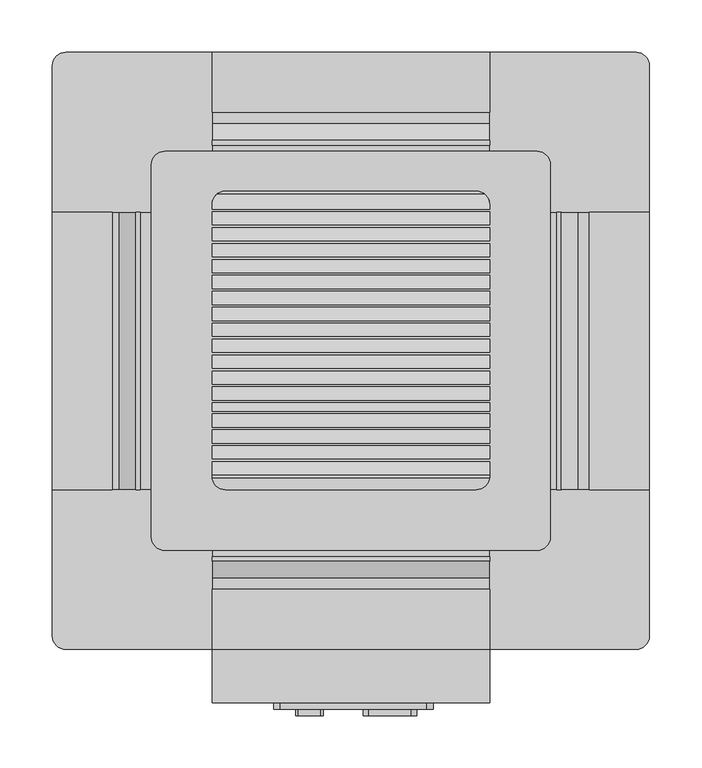
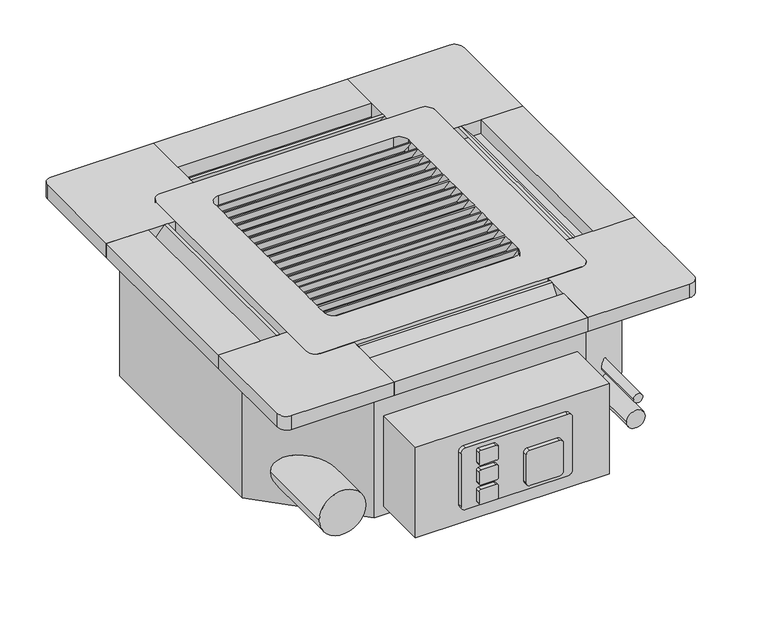
"""IFC4 building model written with IfcOpenShell, lengths in millimetres: proxy geometry, PLFY-P-NCMU-E_4-way_24x24 : PLFY-P12NCMU-E."""

from ifc_helpers import new_model, si_unit, point, frame, frame_2d, origin, place, context, project, spatial, polyline, circle_curve, ellipse_curve, trimmed, segment, composite_curve, outline, extrude, source, transform, mapped, element, save
from ifc_brep_helpers import plane_surface, cylinder_surface, revolved_surface, advanced_brep


def mechanical_equipment_2d84379e(model_context):
    return source(origin(), model_context, "Body", "SolidModel", [
        extrude(outline(polyline([(284.95625, -201.1772913), (227.80625, -201.1772913), (227.80625, 63.9352087), (284.95625, 63.9352087), (284.95625, -201.1772913)])), frame((0.0, 0.0, -1.02e-05), z_axis=(0.0, 0.0, 1.0), x_axis=(1.0, 0.0, 0.0)), (0.0, 0.0, 1.0), 19.84375),
        extrude(outline(polyline([(-284.95625, -201.1772913), (-284.95625, 63.9352087), (-227.80625, 63.9352087), (-227.80625, -201.1772913), (-284.95625, -201.1772913)])), frame((0.0, 0.0, -1.02e-05), z_axis=(0.0, 0.0, 1.0), x_axis=(1.0, 0.0, 0.0)), (0.0, 0.0, 1.0), 19.84375),
        extrude(outline(polyline([(-132.55625, 216.3352087), (132.55625, 216.3352087), (132.55625, 159.1852087), (-132.55625, 159.1852087), (-132.55625, 216.3352087)])), frame((0.0, 0.0, -1.02e-05), z_axis=(0.0, 0.0, 1.0), x_axis=(1.0, 0.0, 0.0)), (0.0, 0.0, 1.0), 19.84375),
        extrude(outline(polyline([(-132.55625, -353.5772913), (-132.55625, -296.4272913), (132.55625, -296.4272913), (132.55625, -353.5772913), (-132.55625, -353.5772913)])), frame((0.0, 0.0, -1.02e-05), z_axis=(0.0, 0.0, 1.0), x_axis=(1.0, 0.0, 0.0)), (0.0, 0.0, 1.0), 19.84375),
        extrude(outline(polyline([(-187.079491, 19.8437398), (-173.1847477, -1.02e-05), (-175.7772913, -1.02e-05), (-189.6720346, 19.8437398), (-187.079491, 19.8437398)])), frame((-132.55625, 0.0, 0.0), z_axis=(1.0, 0.0, 0.0), x_axis=(0.0, 1.0, 0.0)), (0.0, 0.0, 1.0), 265.1125),
        advanced_brep(
        [(-177.8, -259.1210413, -1.02e-05), (-190.5, -246.4210413, -1.02e-05), (-190.5, 109.1789587, -1.02e-05), (-177.8, 121.8789587, -1.02e-05), (177.8, 121.8789587, -1.02e-05), (190.5, 109.1789587, -1.02e-05), (190.5, -246.4210413, -1.02e-05), (177.8, -259.1210413, -1.02e-05), (132.55625, -130.1575084, -1.02e-05), (-132.55625, -130.1575084, -1.02e-05), (-132.55625, -142.7715591, -1.02e-05), (132.55625, -142.7715591, -1.02e-05), (132.55625, -114.9509141, -1.02e-05), (-132.55625, -114.9509141, -1.02e-05), (-132.55625, -127.5649648, -1.02e-05), (132.55625, -127.5649648, -1.02e-05), (132.55625, -104.3814755, -1.02e-05), (-132.55625, -104.3814755, -1.02e-05), (-132.55625, -112.3583705, -1.02e-05), (132.55625, -112.3583705, -1.02e-05), (132.55625, -89.1748812, -1.02e-05), (-132.55625, -89.1748812, -1.02e-05), (-132.55625, -101.7889319, -1.02e-05), (132.55625, -101.7889319, -1.02e-05), (132.55625, -73.9682869, -1.02e-05), (-132.55625, -73.9682869, -1.02e-05), (-132.55625, -86.5823376, -1.02e-05), (132.55625, -86.5823376, -1.02e-05), (132.55625, -58.7616926, -1.02e-05), (-132.55625, -58.7616926, -1.02e-05), (-132.55625, -71.3757433, -1.02e-05), (132.55625, -71.3757433, -1.02e-05), (132.55625, -43.5550983, -1.02e-05), (-132.55625, -43.5550983, -1.02e-05), (-132.55625, -56.169149, -1.02e-05), (132.55625, -56.169149, -1.02e-05), (132.55625, -28.348504, -1.02e-05), (-132.55625, -28.348504, -1.02e-05), (-132.55625, -40.9625547, -1.02e-05), (132.55625, -40.9625547, -1.02e-05), (132.55625, -13.1419097, -1.02e-05), (-132.55625, -13.1419097, -1.02e-05), (-132.55625, -25.7559604, -1.02e-05), (132.55625, -25.7559604, -1.02e-05), (132.55625, 32.4778732, -1.02e-05), (-132.55625, 32.4778732, -1.02e-05), (-132.55625, 19.8638225, -1.02e-05), (132.55625, 19.8638225, -1.02e-05), (132.55625, 47.6844675, -1.02e-05), (-132.55625, 47.6844675, -1.02e-05), (-132.55625, 35.0704168, -1.02e-05), (132.55625, 35.0704168, -1.02e-05), (132.55625, 62.8910618, -1.02e-05), (-132.55625, 62.8910618, -1.02e-05), (-132.55625, 50.2770111, -1.02e-05), (132.55625, 50.2770111, -1.02e-05), (132.55625, 2.0646846, -1.02e-05), (-132.55625, 2.0646846, -1.02e-05), (-132.55625, -10.5493661, -1.02e-05), (132.55625, -10.5493661, -1.02e-05), (-132.55625, 4.6572282, -1.02e-05), (132.55625, 4.6572282, -1.02e-05), (132.55625, 17.2712789, -1.02e-05), (-132.55625, 17.2712789, -1.02e-05), (132.55625, 71.0789587, -1.02e-05), (130.4405727, 78.0976561, -1.02e-05), (-130.4405727, 78.0976561, -1.02e-05), (-132.55625, 71.0789587, -1.02e-05), (-132.55625, 65.4836054, -1.02e-05), (132.55625, 65.4836054, -1.02e-05), (-132.55625, -145.3641027, -1.02e-05), (-132.55625, -157.9781534, -1.02e-05), (132.55625, -157.9781534, -1.02e-05), (132.55625, -145.3641027, -1.02e-05), (-132.55625, -188.4772913, -1.02e-05), (-119.85625, -201.1772913, -1.02e-05), (119.85625, -201.1772913, -1.02e-05), (132.55625, -188.4772913, -1.02e-05), (132.55625, -160.570697, -1.02e-05), (-132.55625, -160.570697, -1.02e-05), (119.85625, 83.7789587, -1.02e-05), (-119.85625, 83.7789587, -1.02e-05), (-128.1576984, 80.6901997, -1.02e-05), (128.1576984, 80.6901997, -1.02e-05), (-177.8, -259.1210413, 19.8437398), (177.8, -259.1210413, 19.8437398), (190.5, -246.4210413, 19.8437398), (190.5, 109.1789587, 19.8437398), (177.8, 121.8789587, 19.8437398), (-177.8, 121.8789587, 19.8437398), (-190.5, 109.1789587, 19.8437398), (-190.5, -246.4210413, 19.8437398), (-132.55625, -144.0522517, 19.8437398), (132.55625, -144.0522517, 19.8437398), (132.55625, -156.6663024, 19.8437398), (-132.55625, -156.6663024, 19.8437398), (-132.55625, -128.8456574, 19.8437398), (132.55625, -128.8456574, 19.8437398), (132.55625, -141.4597081, 19.8437398), (-132.55625, -141.4597081, 19.8437398), (-132.55625, -118.2762188, 19.8437398), (132.55625, -118.2762188, 19.8437398), (132.55625, -126.2531138, 19.8437398), (-132.55625, -126.2531138, 19.8437398), (-132.55625, -103.0696245, 19.8437398), (132.55625, -103.0696245, 19.8437398), (132.55625, -115.6836752, 19.8437398), (-132.55625, -115.6836752, 19.8437398), (-132.55625, -87.8630302, 19.8437398), (132.55625, -87.8630302, 19.8437398), (132.55625, -100.4770809, 19.8437398), (-132.55625, -100.4770809, 19.8437398), (-132.55625, -72.6564359, 19.8437398), (132.55625, -72.6564359, 19.8437398), (132.55625, -85.2704866, 19.8437398), (-132.55625, -85.2704866, 19.8437398), (-132.55625, -57.4498416, 19.8437398), (132.55625, -57.4498416, 19.8437398), (132.55625, -70.0638923, 19.8437398), (-132.55625, -70.0638923, 19.8437398), (-132.55625, -42.2432473, 19.8437398), (132.55625, -42.2432473, 19.8437398), (132.55625, -54.857298, 19.8437398), (-132.55625, -54.857298, 19.8437398), (-132.55625, -27.036653, 19.8437398), (132.55625, -27.036653, 19.8437398), (132.55625, -39.6507037, 19.8437398), (-132.55625, -39.6507037, 19.8437398), (-132.55625, 18.5831298, 19.8437398), (132.55625, 18.5831298, 19.8437398), (132.55625, 5.9690792, 19.8437398), (-132.55625, 5.9690792, 19.8437398), (-132.55625, 33.7897241, 19.8437398), (132.55625, 33.7897241, 19.8437398), (132.55625, 21.1756735, 19.8437398), (-132.55625, 21.1756735, 19.8437398), (-132.55625, 48.9963184, 19.8437398), (132.55625, 48.9963184, 19.8437398), (132.55625, 36.3822678, 19.8437398), (-132.55625, 36.3822678, 19.8437398), (-132.55625, -11.8300587, 19.8437398), (132.55625, -11.8300587, 19.8437398), (132.55625, -24.4441094, 19.8437398), (-132.55625, -24.4441094, 19.8437398), (132.55625, -9.2375151, 19.8437398), (-132.55625, -9.2375151, 19.8437398), (-132.55625, 3.3765356, 19.8437398), (132.55625, 3.3765356, 19.8437398), (-132.55625, 64.2029127, 19.8437398), (132.55625, 64.2029127, 19.8437398), (132.55625, 51.5888621, 19.8437398), (-132.55625, 51.5888621, 19.8437398), (-132.55625, 71.0789587, 19.8437398), (-119.85625, 83.7789587, 19.8437398), (119.85625, 83.7789587, 19.8437398), (132.55625, 71.0789587, 19.8437398), (132.55625, 66.7954564, 19.8437398), (-132.55625, 66.7954564, 19.8437398), (132.55625, -159.258846, 19.8437398), (132.55625, -171.8728967, 19.8437398), (-132.55625, -171.8728967, 19.8437398), (-132.55625, -159.258846, 19.8437398), (132.55625, -188.4772913, 19.8437398), (119.85625, -201.1772913, 19.8437398), (-119.85625, -201.1772913, 19.8437398), (-132.55625, -188.4772913, 19.8437398), (-132.55625, -174.4654403, 19.8437398), (132.55625, -174.4654403, 19.8437398), (132.55625, 71.0789587, 13.7262645), (132.55625, 71.0789587, 10.0237284), (-132.55625, 71.0789587, 10.0237284), (-132.55625, 71.0789587, 13.7262645)],
        [
            (0, 1, circle_curve(frame((-177.8, -246.4210413, -1.02e-05), z_axis=(0.0, 0.0, -1.0), x_axis=(-1.0, 0.0, 0.0)), 12.7)),
            (1, 2),
            (2, 3, circle_curve(frame((-177.8, 109.1789587, -1.02e-05), z_axis=(0.0, 0.0, -1.0), x_axis=(-1.0, 0.0, 0.0)), 12.7)),
            (3, 4),
            (4, 5, circle_curve(frame((177.8, 109.1789587, -1.02e-05), z_axis=(0.0, 0.0, -1.0), x_axis=(-1.0, 0.0, 0.0)), 12.7)),
            (5, 6),
            (6, 7, circle_curve(frame((177.8, -246.4210413, -1.02e-05), z_axis=(0.0, 0.0, -1.0), x_axis=(-1.0, 0.0, 0.0)), 12.7)),
            (7, 0),
            (8, 9),
            (9, 10),
            (10, 11),
            (11, 8),
            (12, 13),
            (13, 14),
            (14, 15),
            (15, 12),
            (16, 17),
            (17, 18),
            (18, 19),
            (19, 16),
            (20, 21),
            (21, 22),
            (22, 23),
            (23, 20),
            (24, 25),
            (25, 26),
            (26, 27),
            (27, 24),
            (28, 29),
            (29, 30),
            (30, 31),
            (31, 28),
            (32, 33),
            (33, 34),
            (34, 35),
            (35, 32),
            (36, 37),
            (37, 38),
            (38, 39),
            (39, 36),
            (40, 41),
            (41, 42),
            (42, 43),
            (43, 40),
            (44, 45),
            (45, 46),
            (46, 47),
            (47, 44),
            (48, 49),
            (49, 50),
            (50, 51),
            (51, 48),
            (52, 53),
            (53, 54),
            (54, 55),
            (55, 52),
            (56, 57),
            (57, 58),
            (58, 59),
            (59, 56),
            (60, 61),
            (61, 62),
            (62, 63),
            (63, 60),
            (64, 65, circle_curve(frame((119.85625, 71.0789587, -1.02e-05), z_axis=(0.0, 0.0, 1.0), x_axis=(-1.0, 0.0, 0.0)), 12.7)),
            (65, 66),
            (66, 67, circle_curve(frame((-119.85625, 71.0789587, -1.02e-05), z_axis=(0.0, 0.0, 1.0), x_axis=(-1.0, 0.0, 0.0)), 12.7)),
            (67, 68),
            (68, 69),
            (69, 64),
            (70, 71),
            (71, 72),
            (72, 73),
            (73, 70),
            (74, 75, circle_curve(frame((-119.85625, -188.4772913, -1.02e-05), z_axis=(0.0, 0.0, 1.0), x_axis=(-1.0, 0.0, 0.0)), 12.7)),
            (75, 76),
            (76, 77, circle_curve(frame((119.85625, -188.4772913, -1.02e-05), z_axis=(0.0, 0.0, 1.0), x_axis=(-1.0, 0.0, 0.0)), 12.7)),
            (77, 78),
            (78, 79),
            (79, 74),
            (80, 81),
            (81, 82, circle_curve(frame((-119.85625, 71.0789587, -1.02e-05), z_axis=(0.0, 0.0, 1.0), x_axis=(-1.0, 0.0, 0.0)), 12.7)),
            (82, 83),
            (83, 80, circle_curve(frame((119.85625, 71.0789587, -1.02e-05), z_axis=(0.0, 0.0, 1.0), x_axis=(-1.0, 0.0, 0.0)), 12.7)),
            (84, 85),
            (85, 86, circle_curve(frame((177.8, -246.4210413, 19.8437398), z_axis=(0.0, 0.0, 1.0), x_axis=(-1.0, 0.0, 0.0)), 12.7)),
            (86, 87),
            (87, 88, circle_curve(frame((177.8, 109.1789587, 19.8437398), z_axis=(0.0, 0.0, 1.0), x_axis=(-1.0, 0.0, 0.0)), 12.7)),
            (88, 89),
            (89, 90, circle_curve(frame((-177.8, 109.1789587, 19.8437398), z_axis=(0.0, 0.0, 1.0), x_axis=(-1.0, 0.0, 0.0)), 12.7)),
            (90, 91),
            (91, 84, circle_curve(frame((-177.8, -246.4210413, 19.8437398), z_axis=(0.0, 0.0, 1.0), x_axis=(-1.0, 0.0, 0.0)), 12.7)),
            (92, 93),
            (93, 94),
            (94, 95),
            (95, 92),
            (96, 97),
            (97, 98),
            (98, 99),
            (99, 96),
            (100, 101),
            (101, 102),
            (102, 103),
            (103, 100),
            (104, 105),
            (105, 106),
            (106, 107),
            (107, 104),
            (108, 109),
            (109, 110),
            (110, 111),
            (111, 108),
            (112, 113),
            (113, 114),
            (114, 115),
            (115, 112),
            (116, 117),
            (117, 118),
            (118, 119),
            (119, 116),
            (120, 121),
            (121, 122),
            (122, 123),
            (123, 120),
            (124, 125),
            (125, 126),
            (126, 127),
            (127, 124),
            (128, 129),
            (129, 130),
            (130, 131),
            (131, 128),
            (132, 133),
            (133, 134),
            (134, 135),
            (135, 132),
            (136, 137),
            (137, 138),
            (138, 139),
            (139, 136),
            (140, 141),
            (141, 142),
            (142, 143),
            (143, 140),
            (144, 145),
            (145, 146),
            (146, 147),
            (147, 144),
            (148, 149),
            (149, 150),
            (150, 151),
            (151, 148),
            (152, 153, circle_curve(frame((-119.85625, 71.0789587, 19.8437398), z_axis=(0.0, 0.0, -1.0), x_axis=(-1.0, 0.0, 0.0)), 12.7)),
            (153, 154),
            (154, 155, circle_curve(frame((119.85625, 71.0789587, 19.8437398), z_axis=(0.0, 0.0, -1.0), x_axis=(-1.0, 0.0, 0.0)), 12.7)),
            (155, 156),
            (156, 157),
            (157, 152),
            (158, 159),
            (159, 160),
            (160, 161),
            (161, 158),
            (162, 163, circle_curve(frame((119.85625, -188.4772913, 19.8437398), z_axis=(0.0, 0.0, -1.0), x_axis=(-1.0, 0.0, 0.0)), 12.7)),
            (163, 164),
            (164, 165, circle_curve(frame((-119.85625, -188.4772913, 19.8437398), z_axis=(0.0, 0.0, -1.0), x_axis=(-1.0, 0.0, 0.0)), 12.7)),
            (165, 166),
            (166, 167),
            (167, 162),
            (155, 168),
            (168, 156),
            (77, 162),
            (167, 78),
            (169, 64),
            (69, 150),
            (149, 169),
            (61, 144),
            (147, 62),
            (141, 56),
            (59, 142),
            (137, 52),
            (55, 138),
            (133, 48),
            (51, 134),
            (129, 44),
            (47, 130),
            (125, 40),
            (43, 126),
            (121, 36),
            (39, 122),
            (117, 32),
            (35, 118),
            (113, 28),
            (31, 114),
            (109, 24),
            (27, 110),
            (105, 20),
            (23, 106),
            (101, 16),
            (19, 102),
            (97, 12),
            (15, 98),
            (93, 8),
            (11, 94),
            (158, 73),
            (72, 159),
            (169, 65, ellipse_curve(frame((119.85625, 71.0789587, 10.0237284), z_axis=(0.0, 0.8191520442889908, 0.5735764363510476), x_axis=(0.0, -0.5735764363510477, 0.8191520442889908)), 22.1417743, 12.7)),
            (154, 80),
            (83, 168, ellipse_curve(frame((119.85625, 71.0789587, 13.7262645), z_axis=(0.0, -0.8191520442889919, -0.573576436351046), x_axis=(0.0, -0.5735764363510462, 0.8191520442889919)), 22.1417743, 12.7)),
            (153, 81),
            (66, 170, ellipse_curve(frame((-119.85625, 71.0789587, 10.0237284), z_axis=(0.0, 0.8191520442889908, 0.5735764363510476), x_axis=(0.0, -0.5735764363510477, 0.8191520442889908)), 22.1417743, 12.7)),
            (170, 67),
            (152, 171),
            (171, 82, ellipse_curve(frame((-119.85625, 71.0789587, 13.7262645), z_axis=(0.0, -0.8191520442889919, -0.573576436351046), x_axis=(0.0, -0.5735764363510462, 0.8191520442889919)), 22.1417743, 12.7)),
            (157, 171),
            (170, 148),
            (151, 68),
            (165, 74),
            (79, 166),
            (145, 60),
            (63, 146),
            (57, 140),
            (143, 58),
            (53, 136),
            (139, 54),
            (49, 132),
            (135, 50),
            (45, 128),
            (131, 46),
            (41, 124),
            (127, 42),
            (37, 120),
            (123, 38),
            (33, 116),
            (119, 34),
            (29, 112),
            (115, 30),
            (25, 108),
            (111, 26),
            (21, 104),
            (107, 22),
            (17, 100),
            (103, 18),
            (13, 96),
            (99, 14),
            (9, 92),
            (95, 10),
            (70, 161),
            (160, 71),
            (164, 75),
            (163, 76),
            (0, 84),
            (91, 1),
            (90, 2),
            (89, 3),
            (88, 4),
            (87, 5),
            (86, 6),
            (85, 7),
        ],
        [
            plane_surface(frame((132.55625, 71.0789587, -1.02e-05), z_axis=(0.0, 0.0, -1.0), x_axis=(0.0, 1.0, 0.0))),
            plane_surface(frame((132.55625, 71.0789587, 19.8437398), z_axis=(0.0, 0.0, 1.0), x_axis=(0.0, -1.0, 0.0))),
            plane_surface(frame((132.55625, -188.4772913, -1.02e-05), z_axis=(-1.0, 0.0, 0.0), x_axis=(0.0, 0.0, 1.0))),
            revolved_surface(polyline([(107.15625, 71.0789587, 28.161208082030438), (107.15625, 71.0789587, -8.113751282030439)]), (119.85625, 71.0789587, 19.8437398), (0.0, 0.0, 1.0)),
            revolved_surface(polyline([(107.15625, 71.0789587, 31.863744182030462), (107.15625, 71.0789587, -4.411215182030464)]), (119.85625, 71.0789587, 19.8437398), (0.0, 0.0, 1.0)),
            plane_surface(frame((119.85625, 83.7789587, -1.02e-05), z_axis=(0.0, -1.0, 0.0), x_axis=(0.0, 0.0, 1.0))),
            revolved_surface(polyline([(-132.55625, 71.0789587, 28.161208082030438), (-132.55625, 71.0789587, -8.113751282030439)]), (-119.85625, 71.0789587, 19.8437398), (0.0, 0.0, 1.0)),
            revolved_surface(polyline([(-132.55625, 71.0789587, 31.863744182030462), (-132.55625, 71.0789587, -4.411215182030464)]), (-119.85625, 71.0789587, 19.8437398), (0.0, 0.0, 1.0)),
            plane_surface(frame((-132.55625, 71.0789587, -1.02e-05), z_axis=(1.0, 0.0, 0.0), x_axis=(0.0, 0.0, 1.0))),
            revolved_surface(polyline([(-132.55625, -188.4772913, 19.8437398), (-132.55625, -188.4772913, -1.0199999998405929e-05)]), (-119.85625, -188.4772913, 19.8437398), (0.0, 0.0, 1.0)),
            plane_surface(frame((-119.85625, -201.1772913, -1.02e-05), z_axis=(0.0, 1.0, 0.0), x_axis=(0.0, 0.0, 1.0))),
            revolved_surface(polyline([(107.15625, -188.4772913, 19.8437398), (107.15625, -188.4772913, -1.0199999998405929e-05)]), (119.85625, -188.4772913, 19.8437398), (0.0, 0.0, 1.0)),
            cylinder_surface(frame((-177.8, -246.4210413, -1.02e-05), z_axis=(0.0, 0.0, -1.0), x_axis=(-1.0, 0.0, 0.0)), 12.7),
            plane_surface(frame((-190.5, -246.4210413, -1.02e-05), z_axis=(-1.0, 0.0, 0.0), x_axis=(0.0, 0.0, 1.0))),
            cylinder_surface(frame((-177.8, 109.1789587, -1.02e-05), z_axis=(0.0, 0.0, -1.0), x_axis=(-1.0, 0.0, 0.0)), 12.7),
            plane_surface(frame((-177.8, 121.8789587, -1.02e-05), z_axis=(0.0, 1.0, 0.0), x_axis=(0.0, 0.0, 1.0))),
            cylinder_surface(frame((177.8, 109.1789587, -1.02e-05), z_axis=(0.0, 0.0, -1.0), x_axis=(-1.0, 0.0, 0.0)), 12.7),
            plane_surface(frame((190.5, 109.1789587, -1.02e-05), z_axis=(1.0, 0.0, 0.0), x_axis=(0.0, 0.0, 1.0))),
            cylinder_surface(frame((177.8, -246.4210413, -1.02e-05), z_axis=(0.0, 0.0, -1.0), x_axis=(-1.0, 0.0, 0.0)), 12.7),
            plane_surface(frame((177.8, -259.1210413, -1.02e-05), z_axis=(0.0, -1.0, 0.0), x_axis=(0.0, 0.0, 1.0))),
            plane_surface(frame((-132.55625, 66.7954564, 19.8437398), z_axis=(0.0, 0.8191520442889919, 0.573576436351046), x_axis=(1.0, 0.0, 0.0))),
            plane_surface(frame((-132.55625, 78.0976561, -1.02e-05), z_axis=(0.0, -0.8191520442889908, -0.5735764363510476), x_axis=(1.0, 0.0, 0.0))),
            plane_surface(frame((-132.55625, -9.2375151, 19.8437398), z_axis=(0.0, 0.8191520442889919, 0.573576436351046), x_axis=(1.0, 0.0, 0.0))),
            plane_surface(frame((-132.55625, 2.0646846, -1.02e-05), z_axis=(0.0, -0.8191520442889908, -0.5735764363510476), x_axis=(1.0, 0.0, 0.0))),
            plane_surface(frame((-132.55625, 51.5888621, 19.8437398), z_axis=(0.0, 0.8191520442889909, 0.5735764363510475), x_axis=(1.0, 0.0, 0.0))),
            plane_surface(frame((-132.55625, 62.8910618, -1.02e-05), z_axis=(0.0, -0.8191520442889917, -0.5735764363510462), x_axis=(1.0, 0.0, 0.0))),
            plane_surface(frame((-132.55625, 36.3822678, 19.8437398), z_axis=(0.0, 0.8191520442889899, 0.5735764363510489), x_axis=(1.0, 0.0, 0.0))),
            plane_surface(frame((-132.55625, 47.6844675, -1.02e-05), z_axis=(0.0, -0.8191520442889901, -0.5735764363510485), x_axis=(1.0, 0.0, 0.0))),
            plane_surface(frame((-132.55625, 21.1756735, 19.8437398), z_axis=(0.0, 0.8191520442889908, 0.5735764363510477), x_axis=(1.0, 0.0, 0.0))),
            plane_surface(frame((-132.55625, 32.4778732, -1.02e-05), z_axis=(0.0, -0.8191520442889919, -0.5735764363510462), x_axis=(1.0, 0.0, 0.0))),
            plane_surface(frame((-132.55625, 5.9690792, 19.8437398), z_axis=(0.0, 0.8191520442889905, 0.5735764363510482), x_axis=(1.0, 0.0, 0.0))),
            plane_surface(frame((-132.55625, 17.2712789, -1.02e-05), z_axis=(0.0, -0.8191520442889922, -0.5735764363510455), x_axis=(1.0, 0.0, 0.0))),
            plane_surface(frame((-132.55625, -24.4441094, 19.8437398), z_axis=(0.0, 0.8191520442889909, 0.5735764363510475), x_axis=(1.0, 0.0, 0.0))),
            plane_surface(frame((-132.55625, -13.1419097, -1.02e-05), z_axis=(0.0, -0.8191520442889917, -0.5735764363510462), x_axis=(1.0, 0.0, 0.0))),
            plane_surface(frame((-132.55625, -39.6507037, 19.8437398), z_axis=(0.0, 0.8191520442889902, 0.5735764363510484), x_axis=(1.0, 0.0, 0.0))),
            plane_surface(frame((-132.55625, -28.348504, -1.02e-05), z_axis=(0.0, -0.8191520442889924, -0.5735764363510453), x_axis=(1.0, 0.0, 0.0))),
            plane_surface(frame((-132.55625, -54.857298, 19.8437398), z_axis=(0.0, 0.8191520442889916, 0.5735764363510465), x_axis=(1.0, 0.0, 0.0))),
            plane_surface(frame((-132.55625, -43.5550983, -1.02e-05), z_axis=(0.0, -0.8191520442889911, -0.5735764363510472), x_axis=(1.0, 0.0, 0.0))),
            plane_surface(frame((-132.55625, -70.0638923, 19.8437398), z_axis=(0.0, 0.8191520442889899, 0.5735764363510489), x_axis=(1.0, 0.0, 0.0))),
            plane_surface(frame((-132.55625, -58.7616926, -1.02e-05), z_axis=(0.0, -0.8191520442889901, -0.5735764363510485), x_axis=(1.0, 0.0, 0.0))),
            plane_surface(frame((-132.55625, -85.2704866, 19.8437398), z_axis=(0.0, 0.8191520442889914, 0.5735764363510468), x_axis=(1.0, 0.0, 0.0))),
            plane_surface(frame((-132.55625, -73.9682869, -1.02e-05), z_axis=(0.0, -0.8191520442889915, -0.5735764363510467), x_axis=(1.0, 0.0, 0.0))),
            plane_surface(frame((-132.55625, -100.4770809, 19.8437398), z_axis=(0.0, 0.8191520442889907, 0.5735764363510477), x_axis=(1.0, 0.0, 0.0))),
            plane_surface(frame((-132.55625, -89.1748812, -1.02e-05), z_axis=(0.0, -0.8191520442889921, -0.5735764363510457), x_axis=(1.0, 0.0, 0.0))),
            plane_surface(frame((-132.55625, -115.6836752, 19.8437398), z_axis=(0.0, 0.819152044288992, 0.5735764363510459), x_axis=(1.0, 0.0, 0.0))),
            plane_surface(frame((-132.55625, -104.3814755, -1.02e-05), z_axis=(0.0, -0.8191520442889908, -0.5735764363510476), x_axis=(1.0, 0.0, 0.0))),
            plane_surface(frame((-132.55625, -126.2531138, 19.8437398), z_axis=(0.0, 0.8191520442889881, 0.5735764363510515), x_axis=(1.0, 0.0, 0.0))),
            plane_surface(frame((-132.55625, -114.9509141, -1.02e-05), z_axis=(0.0, -0.8191520442889907, -0.5735764363510477), x_axis=(1.0, 0.0, 0.0))),
            plane_surface(frame((-132.55625, -141.4597081, 19.8437398), z_axis=(0.0, 0.8191520442889891, 0.5735764363510499), x_axis=(1.0, 0.0, 0.0))),
            plane_surface(frame((-132.55625, -130.1575084, -1.02e-05), z_axis=(0.0, -0.819152044288991, -0.5735764363510474), x_axis=(1.0, 0.0, 0.0))),
            plane_surface(frame((-132.55625, -156.6663024, 19.8437398), z_axis=(0.0, 0.8191520442889885, 0.5735764363510508), x_axis=(1.0, 0.0, 0.0))),
            plane_surface(frame((-132.55625, -145.3641027, -1.02e-05), z_axis=(0.0, -0.819152044288991, -0.5735764363510474), x_axis=(1.0, 0.0, 0.0))),
            plane_surface(frame((-132.55625, -171.8728967, 19.8437398), z_axis=(0.0, 0.8191520442889885, 0.5735764363510508), x_axis=(1.0, 0.0, 0.0))),
            plane_surface(frame((-132.55625, -160.570697, -1.02e-05), z_axis=(0.0, -0.819152044288991, -0.5735764363510474), x_axis=(1.0, 0.0, 0.0))),
        ],
        [
            (0, [[1, 2, 3, 4, 5, 6, 7, 8], [9, 10, 11, 12], [13, 14, 15, 16], [17, 18, 19, 20], [21, 22, 23, 24], [25, 26, 27, 28], [29, 30, 31, 32], [33, 34, 35, 36], [37, 38, 39, 40], [41, 42, 43, 44], [45, 46, 47, 48], [49, 50, 51, 52], [53, 54, 55, 56], [57, 58, 59, 60], [61, 62, 63, 64], [65, 66, 67, 68, 69, 70], [71, 72, 73, 74], [75, 76, 77, 78, 79, 80], [81, 82, 83, 84]]),
            (1, [[85, 86, 87, 88, 89, 90, 91, 92], [93, 94, 95, 96], [97, 98, 99, 100], [101, 102, 103, 104], [105, 106, 107, 108], [109, 110, 111, 112], [113, 114, 115, 116], [117, 118, 119, 120], [121, 122, 123, 124], [125, 126, 127, 128], [129, 130, 131, 132], [133, 134, 135, 136], [137, 138, 139, 140], [141, 142, 143, 144], [145, 146, 147, 148], [149, 150, 151, 152], [153, 154, 155, 156, 157, 158], [159, 160, 161, 162], [163, 164, 165, 166, 167, 168]]),
            (2, [[-156, 169, 170]]),
            (2, [[171, -168, 172, -78]]),
            (2, [[173, -70, 174, -150, 175]]),
            (2, [[176, -148, 177, -62]]),
            (2, [[178, -60, 179, -142]]),
            (2, [[180, -56, 181, -138]]),
            (2, [[182, -52, 183, -134]]),
            (2, [[184, -48, 185, -130]]),
            (2, [[186, -44, 187, -126]]),
            (2, [[188, -40, 189, -122]]),
            (2, [[190, -36, 191, -118]]),
            (2, [[192, -32, 193, -114]]),
            (2, [[194, -28, 195, -110]]),
            (2, [[196, -24, 197, -106]]),
            (2, [[198, -20, 199, -102]]),
            (2, [[200, -16, 201, -98]]),
            (2, [[202, -12, 203, -94]]),
            (2, [[204, -73, 205, -159]]),
            (3, [[-65, -173, 206]]),
            (4, [[-155, 207, -84, 208, -169]]),
            (5, [[-81, -207, -154, 209]]),
            (6, [[-67, 210, 211]]),
            (7, [[-153, 212, 213, -82, -209]]),
            (8, [[-158, 214, -212]]),
            (8, [[-211, 215, -152, 216, -68]]),
            (8, [[217, -80, 218, -166]]),
            (8, [[219, -64, 220, -146]]),
            (8, [[221, -144, 222, -58]]),
            (8, [[223, -140, 224, -54]]),
            (8, [[225, -136, 226, -50]]),
            (8, [[227, -132, 228, -46]]),
            (8, [[229, -128, 230, -42]]),
            (8, [[231, -124, 232, -38]]),
            (8, [[233, -120, 234, -34]]),
            (8, [[235, -116, 236, -30]]),
            (8, [[237, -112, 238, -26]]),
            (8, [[239, -108, 240, -22]]),
            (8, [[241, -104, 242, -18]]),
            (8, [[243, -100, 244, -14]]),
            (8, [[245, -96, 246, -10]]),
            (8, [[247, -161, 248, -71]]),
            (9, [[-75, -217, -165, 249]]),
            (10, [[-76, -249, -164, 250]]),
            (11, [[-77, -250, -163, -171]]),
            (12, [[-1, 251, -92, 252]]),
            (13, [[-2, -252, -91, 253]]),
            (14, [[-3, -253, -90, 254]]),
            (15, [[-4, -254, -89, 255]]),
            (16, [[-5, -255, -88, 256]]),
            (17, [[-6, -256, -87, 257]]),
            (18, [[-7, -257, -86, 258]]),
            (19, [[-8, -258, -85, -251]]),
            (20, [[-157, -170, -208, -83, -213, -214]]),
            (21, [[-149, -215, -210, -66, -206, -175]]),
            (22, [[-145, -176, -61, -219]]),
            (23, [[-57, -178, -141, -221]]),
            (24, [[-151, -174, -69, -216]]),
            (25, [[-53, -180, -137, -223]]),
            (26, [[-139, -181, -55, -224]]),
            (27, [[-49, -182, -133, -225]]),
            (28, [[-135, -183, -51, -226]]),
            (29, [[-45, -184, -129, -227]]),
            (30, [[-131, -185, -47, -228]]),
            (31, [[-63, -177, -147, -220]]),
            (32, [[-143, -179, -59, -222]]),
            (33, [[-41, -186, -125, -229]]),
            (34, [[-127, -187, -43, -230]]),
            (35, [[-37, -188, -121, -231]]),
            (36, [[-123, -189, -39, -232]]),
            (37, [[-33, -190, -117, -233]]),
            (38, [[-119, -191, -35, -234]]),
            (39, [[-29, -192, -113, -235]]),
            (40, [[-115, -193, -31, -236]]),
            (41, [[-25, -194, -109, -237]]),
            (42, [[-111, -195, -27, -238]]),
            (43, [[-21, -196, -105, -239]]),
            (44, [[-107, -197, -23, -240]]),
            (45, [[-17, -198, -101, -241]]),
            (46, [[-103, -199, -19, -242]]),
            (47, [[-13, -200, -97, -243]]),
            (48, [[-99, -201, -15, -244]]),
            (49, [[-9, -202, -93, -245]]),
            (50, [[-95, -203, -11, -246]]),
            (51, [[-74, -204, -162, -247]]),
            (52, [[-160, -205, -72, -248]]),
            (53, [[-79, -172, -167, -218]]),
        ],
    ),
        advanced_brep(
        [(259.55625, 76.6352087, -188.1187602), (259.55625, -213.8772913, -188.1187602), (145.25625, -328.1772913, -188.1187602), (-145.25625, -328.1772913, -188.1187602), (-259.55625, -213.8772913, -188.1187602), (-259.55625, 76.6352087, -188.1187602), (-145.25625, 190.9352087, -188.1187602), (145.25625, 190.9352087, -188.1187602), (259.55625, 76.6352087, -1.02e-05), (145.25625, 190.9352087, -1.02e-05), (-145.25625, 190.9352087, -1.02e-05), (-259.55625, 76.6352087, -1.02e-05), (-259.55625, -213.8772913, -1.02e-05), (-145.25625, -328.1772913, -1.02e-05), (145.25625, -328.1772913, -1.02e-05), (259.55625, -213.8772913, -1.02e-05), (195.2625, -278.1710413, -120.6500102), (207.9625, -265.4710413, -120.6500102), (185.7375, -287.6960413, -150.0187602), (211.1375, -262.2960413, -150.0187602), (-234.95, -238.4835413, -144.6440338), (-171.45, -301.9835413, -144.6440338), (207.9625, -353.5772913, -120.6500102), (195.2625, -353.5772913, -120.6500102), (211.1375, -353.5772913, -150.0187602), (185.7375, -353.5772913, -150.0187602), (-171.45, -353.5772913, -144.6440338), (-234.95, -353.5772913, -144.6440338)],
        [
            (0, 1),
            (1, 2),
            (2, 3),
            (3, 4),
            (4, 5),
            (5, 6),
            (6, 7),
            (7, 0),
            (8, 9),
            (9, 10),
            (10, 11),
            (11, 12),
            (12, 13),
            (13, 14),
            (14, 15),
            (15, 8),
            (0, 8),
            (15, 1),
            (14, 2),
            (16, 17, ellipse_curve(frame((201.6125, -271.8210413, -120.6500102), z_axis=(-0.7071067811865646, 0.7071067811865305, 0.0), x_axis=(-0.7071067811865305, -0.7071067811865646, 0.0)), 8.9802561, 6.35)),
            (17, 16, ellipse_curve(frame((201.6125, -271.8210413, -120.6500102), z_axis=(-0.7071067811865646, 0.7071067811865305, 0.0), x_axis=(-0.7071067811865305, -0.7071067811865646, 0.0)), 8.9802561, 6.35)),
            (18, 19, ellipse_curve(frame((198.4375, -274.9960413, -150.0187602), z_axis=(-0.7071067811865646, 0.7071067811865305, 0.0), x_axis=(-0.7071067811865305, -0.7071067811865646, 0.0)), 17.9605122, 12.7)),
            (19, 18, ellipse_curve(frame((198.4375, -274.9960413, -150.0187602), z_axis=(-0.7071067811865646, 0.7071067811865305, 0.0), x_axis=(-0.7071067811865305, -0.7071067811865646, 0.0)), 17.9605122, 12.7)),
            (13, 3),
            (12, 4),
            (20, 21, ellipse_curve(frame((-203.2, -270.2335413, -144.6440338), z_axis=(0.7071067811865317, 0.7071067811865633, 0.0), x_axis=(0.7071067811865633, -0.7071067811865318, 0.0)), 44.9012806, 31.75)),
            (21, 20, ellipse_curve(frame((-203.2, -270.2335413, -144.6440338), z_axis=(0.7071067811865317, 0.7071067811865633, 0.0), x_axis=(0.7071067811865633, -0.7071067811865318, 0.0)), 44.9012806, 31.75)),
            (11, 5),
            (10, 6),
            (9, 7),
            (22, 23, circle_curve(frame((201.6125, -353.5772913, -120.6500102), z_axis=(0.0, -1.0, 0.0), x_axis=(-1.0, 0.0, 0.0)), 6.35)),
            (23, 22, circle_curve(frame((201.6125, -353.5772913, -120.6500102), z_axis=(0.0, -1.0, 0.0), x_axis=(-1.0, 0.0, 0.0)), 6.35)),
            (24, 25, circle_curve(frame((198.4375, -353.5772913, -150.0187602), z_axis=(0.0, -1.0, 0.0), x_axis=(-1.0, 0.0, 0.0)), 12.7)),
            (25, 24, circle_curve(frame((198.4375, -353.5772913, -150.0187602), z_axis=(0.0, -1.0, 0.0), x_axis=(-1.0, 0.0, 0.0)), 12.7)),
            (22, 17),
            (16, 23),
            (24, 19),
            (18, 25),
            (26, 27, circle_curve(frame((-203.2, -353.5772913, -144.6440338), z_axis=(0.0, -1.0, 0.0), x_axis=(-1.0, 0.0, 0.0)), 31.75)),
            (27, 26, circle_curve(frame((-203.2, -353.5772913, -144.6440338), z_axis=(0.0, -1.0, 0.0), x_axis=(-1.0, 0.0, 0.0)), 31.75)),
            (26, 21),
            (20, 27),
        ],
        [
            plane_surface(frame((259.55625, -213.8772913, -188.1187602), z_axis=(0.0, 0.0, -1.0), x_axis=(0.0, -1.0, 0.0))),
            plane_surface(frame((259.55625, -213.8772913, -1.02e-05), z_axis=(0.0, 0.0, 1.0), x_axis=(0.0, 1.0, 0.0))),
            plane_surface(frame((259.55625, 76.6352087, -188.1187602), z_axis=(1.0, 0.0, 0.0), x_axis=(0.0, 0.0, 1.0))),
            plane_surface(frame((259.55625, -213.8772913, -188.1187602), z_axis=(0.7071067811865646, -0.7071067811865305, 0.0), x_axis=(0.0, 0.0, 1.0))),
            plane_surface(frame((145.25625, -328.1772913, -188.1187602), z_axis=(0.0, -1.0, 0.0), x_axis=(0.0, 0.0, 1.0))),
            plane_surface(frame((-145.25625, -328.1772913, -188.1187602), z_axis=(-0.7071067811865317, -0.7071067811865633, 0.0), x_axis=(0.0, 0.0, 1.0))),
            plane_surface(frame((-259.55625, -213.8772913, -188.1187602), z_axis=(-1.0, 0.0, 0.0), x_axis=(0.0, 0.0, 1.0))),
            plane_surface(frame((-259.55625, 76.6352087, -188.1187602), z_axis=(-0.707106781186534, 0.7071067811865611, 0.0), x_axis=(0.0, 0.0, 1.0))),
            plane_surface(frame((-145.25625, 190.9352087, -188.1187602), z_axis=(0.0, 1.0, 0.0), x_axis=(0.0, 0.0, 1.0))),
            plane_surface(frame((145.25625, 190.9352087, -188.1187602), z_axis=(0.7071067811865633, 0.7071067811865317, 0.0), x_axis=(0.0, 0.0, 1.0))),
            plane_surface(frame((195.2625, -353.5772913, -120.6500102), z_axis=(0.0, -1.0, 0.0), x_axis=(0.0, 0.0, -1.0))),
            cylinder_surface(frame((201.6125, -239.2772913, -120.6500102), z_axis=(0.0, -1.0, 0.0), x_axis=(-1.0, 0.0, 0.0)), 6.35),
            cylinder_surface(frame((198.4375, -68.6210413, -150.0187602), z_axis=(0.0, -1.0, 0.0), x_axis=(-1.0, 0.0, 0.0)), 12.7),
            plane_surface(frame((-234.95, -353.5772913, -144.6440338), z_axis=(0.0, -1.0, 0.0), x_axis=(0.0, 0.0, -1.0))),
            cylinder_surface(frame((-203.2, -201.1772913, -144.6440338), z_axis=(0.0, -1.0, 0.0), x_axis=(-1.0, 0.0, 0.0)), 31.75),
        ],
        [
            (0, [[1, 2, 3, 4, 5, 6, 7, 8]]),
            (1, [[9, 10, 11, 12, 13, 14, 15, 16]]),
            (2, [[-1, 17, -16, 18]]),
            (3, [[-2, -18, -15, 19], [20, 21], [22, 23]]),
            (4, [[-3, -19, -14, 24]]),
            (5, [[-4, -24, -13, 25], [26, 27]]),
            (6, [[-5, -25, -12, 28]]),
            (7, [[-6, -28, -11, 29]]),
            (8, [[-7, -29, -10, 30]]),
            (9, [[-8, -30, -9, -17]]),
            (10, [[31, 32]]),
            (10, [[33, 34]]),
            (11, [[-31, 35, -20, 36]]),
            (11, [[-32, -36, -21, -35]]),
            (12, [[-33, 37, -22, 38]]),
            (12, [[-34, -38, -23, -37]]),
            (13, [[39, 40]]),
            (14, [[-39, 41, -26, 42]]),
            (14, [[-40, -42, -27, -41]]),
        ],
    ),
        extrude(outline(polyline([(132.55625, -328.1772913), (132.55625, -404.3772913), (-132.55625, -404.3772913), (-132.55625, -328.1772913), (132.55625, -328.1772913)])), frame((0.0, 0.0, -175.4187602), z_axis=(0.0, 0.0, 1.0), x_axis=(1.0, 0.0, 0.0)), (0.0, 0.0, 1.0), 130.96875),
        extrude(outline(composite_curve([segment(trimmed(circle_curve(frame_2d((0.0, -63.5)), 63.5), [point((0.0, -127.0))], [point((0.0, 0.0))], False, "CARTESIAN"), True, "CONTINUOUS"), segment(trimmed(circle_curve(frame_2d((0.0, -63.5)), 63.5), [point((0.0, 0.0))], [point((0.0, -127.0))], False, "CARTESIAN"), True, "CONTINUOUS")], self_intersect=False)), frame((247.3075306, 88.8839281, -94.0593852), z_axis=(0.7071067811865633, 0.7071067811865318, 0.0), x_axis=(0.0, 0.0, 1.0)), (0.0, 0.0, 1.0), 6.35),
        extrude(outline(composite_curve([segment(polyline([(-119.7652463, -50.0244022), (-119.7652463, -28.8416002)]), True, "CONTINUOUS"), segment(trimmed(circle_curve(frame_2d((-117.1173961, -28.8416002)), 2.6478502), [point((-119.7652463, -28.8416002))], [point((-117.1173961, -26.19375))], False, "CARTESIAN"), True, "CONTINUOUS"), segment(polyline([(-117.1173961, -26.19375), (-101.0393289, -26.19375)]), True, "CONTINUOUS"), segment(trimmed(circle_curve(frame_2d((-101.0393289, -28.8416002)), 2.6478502), [point((-101.0393289, -26.19375))], [point((-98.3914786, -28.8416002))], False, "CARTESIAN"), True, "CONTINUOUS"), segment(polyline([(-98.3914786, -28.8416002), (-98.3914786, -50.0244022)]), True, "CONTINUOUS"), segment(trimmed(circle_curve(frame_2d((-101.0393289, -50.0244022)), 2.6478502), [point((-98.3914786, -50.0244022))], [point((-101.0393289, -52.6722525))], False, "CARTESIAN"), True, "CONTINUOUS"), segment(polyline([(-101.0393289, -52.6722525), (-117.1173961, -52.6722525)]), True, "CONTINUOUS"), segment(trimmed(circle_curve(frame_2d((-117.1173961, -50.0244022)), 2.6478502), [point((-117.1173961, -52.6722525))], [point((-119.7652463, -50.0244022))], False, "CARTESIAN"), True, "CONTINUOUS")], self_intersect=False)), frame((0.0, -416.8418946, 0.0), z_axis=(0.0, 1.0, 0.0), x_axis=(0.0, 0.0, 1.0)), (0.0, 0.0, 1.0), 6.1146033),
        extrude(outline(composite_curve([segment(polyline([(-91.389546, -50.0244022), (-91.389546, -28.8416002)]), True, "CONTINUOUS"), segment(trimmed(circle_curve(frame_2d((-88.7416958, -28.8416002)), 2.6478502), [point((-91.389546, -28.8416002))], [point((-88.7416958, -26.19375))], False, "CARTESIAN"), True, "CONTINUOUS"), segment(polyline([(-88.7416958, -26.19375), (-72.6636286, -26.19375)]), True, "CONTINUOUS"), segment(trimmed(circle_curve(frame_2d((-72.6636286, -28.8416002)), 2.6478502), [point((-72.6636286, -26.19375))], [point((-70.0157783, -28.8416002))], False, "CARTESIAN"), True, "CONTINUOUS"), segment(polyline([(-70.0157783, -28.8416002), (-70.0157783, -50.0244022)]), True, "CONTINUOUS"), segment(trimmed(circle_curve(frame_2d((-72.6636286, -50.0244022)), 2.6478502), [point((-70.0157783, -50.0244022))], [point((-72.6636286, -52.6722525))], False, "CARTESIAN"), True, "CONTINUOUS"), segment(polyline([(-72.6636286, -52.6722525), (-88.7416958, -52.6722525)]), True, "CONTINUOUS"), segment(trimmed(circle_curve(frame_2d((-88.7416958, -50.0244022)), 2.6478502), [point((-88.7416958, -52.6722525))], [point((-91.389546, -50.0244022))], False, "CARTESIAN"), True, "CONTINUOUS")], self_intersect=False)), frame((0.0, -416.8418946, 0.0), z_axis=(0.0, 1.0, 0.0), x_axis=(0.0, 0.0, 1.0)), (0.0, 0.0, 1.0), 6.1146033),
        extrude(outline(composite_curve([segment(polyline([(-148.1409467, -50.0244022), (-148.1409467, -28.8416002)]), True, "CONTINUOUS"), segment(trimmed(circle_curve(frame_2d((-145.4930964, -28.8416002)), 2.6478502), [point((-148.1409467, -28.8416002))], [point((-145.4930964, -26.19375))], False, "CARTESIAN"), True, "CONTINUOUS"), segment(polyline([(-145.4930964, -26.19375), (-129.4150292, -26.19375)]), True, "CONTINUOUS"), segment(trimmed(circle_curve(frame_2d((-129.4150292, -28.8416002)), 2.6478502), [point((-129.4150292, -26.19375))], [point((-126.767179, -28.8416002))], False, "CARTESIAN"), True, "CONTINUOUS"), segment(polyline([(-126.767179, -28.8416002), (-126.767179, -50.0244022)]), True, "CONTINUOUS"), segment(trimmed(circle_curve(frame_2d((-129.4150292, -50.0244022)), 2.6478502), [point((-126.767179, -50.0244022))], [point((-129.4150292, -52.6722525))], False, "CARTESIAN"), True, "CONTINUOUS"), segment(polyline([(-129.4150292, -52.6722525), (-145.4930964, -52.6722525)]), True, "CONTINUOUS"), segment(trimmed(circle_curve(frame_2d((-145.4930964, -50.0244022)), 2.6478502), [point((-145.4930964, -52.6722525))], [point((-148.1409467, -50.0244022))], False, "CARTESIAN"), True, "CONTINUOUS")], self_intersect=False)), frame((0.0, -416.8418946, 0.0), z_axis=(0.0, 1.0, 0.0), x_axis=(0.0, 0.0, 1.0)), (0.0, 0.0, 1.0), 6.1146033),
        extrude(outline(composite_curve([segment(polyline([(-144.2230964, 16.98625), (-144.2230964, 57.62625)]), True, "CONTINUOUS"), segment(trimmed(circle_curve(frame_2d((-139.1430964, 57.62625)), 5.08), [point((-144.2230964, 57.62625))], [point((-139.1430964, 62.70625))], False, "CARTESIAN"), True, "CONTINUOUS"), segment(polyline([(-139.1430964, 62.70625), (-98.5030964, 62.70625)]), True, "CONTINUOUS"), segment(trimmed(circle_curve(frame_2d((-98.5030964, 57.62625)), 5.08), [point((-98.5030964, 62.70625))], [point((-93.4230964, 57.62625))], False, "CARTESIAN"), True, "CONTINUOUS"), segment(polyline([(-93.4230964, 57.62625), (-93.4230964, 16.98625)]), True, "CONTINUOUS"), segment(trimmed(circle_curve(frame_2d((-98.5030964, 16.98625)), 5.08), [point((-93.4230964, 16.98625))], [point((-98.5030964, 11.90625))], False, "CARTESIAN"), True, "CONTINUOUS"), segment(polyline([(-98.5030964, 11.90625), (-139.1430964, 11.90625)]), True, "CONTINUOUS"), segment(trimmed(circle_curve(frame_2d((-139.1430964, 16.98625)), 5.08), [point((-139.1430964, 11.90625))], [point((-144.2230964, 16.98625))], False, "CARTESIAN"), True, "CONTINUOUS")], self_intersect=False)), frame((0.0, -416.8418946, 0.0), z_axis=(0.0, 1.0, 0.0), x_axis=(0.0, 0.0, 1.0)), (0.0, 0.0, 1.0), 6.1146033),
        extrude(outline(composite_curve([segment(polyline([(-153.0807513, -67.46875), (-153.0807513, 72.23125)]), True, "CONTINUOUS"), segment(trimmed(circle_curve(frame_2d((-146.7307513, 72.23125)), 6.35), [point((-153.0807513, 72.23125))], [point((-146.7307513, 78.58125))], False, "CARTESIAN"), True, "CONTINUOUS"), segment(polyline([(-146.7307513, 78.58125), (-70.5307513, 78.58125)]), True, "CONTINUOUS"), segment(trimmed(circle_curve(frame_2d((-70.5307513, 72.23125)), 6.35), [point((-70.5307513, 78.58125))], [point((-64.1807513, 72.23125))], False, "CARTESIAN"), True, "CONTINUOUS"), segment(polyline([(-64.1807513, 72.23125), (-64.1807513, -67.46875)]), True, "CONTINUOUS"), segment(trimmed(circle_curve(frame_2d((-70.5307513, -67.46875)), 6.35), [point((-64.1807513, -67.46875))], [point((-70.5307513, -73.81875))], False, "CARTESIAN"), True, "CONTINUOUS"), segment(polyline([(-70.5307513, -73.81875), (-146.7307513, -73.81875)]), True, "CONTINUOUS"), segment(trimmed(circle_curve(frame_2d((-146.7307513, -67.46875)), 6.35), [point((-146.7307513, -73.81875))], [point((-153.0807513, -67.46875))], False, "CARTESIAN"), True, "CONTINUOUS")], self_intersect=False)), frame((0.0, -410.7272913, 0.0), z_axis=(0.0, 1.0, 0.0), x_axis=(0.0, 0.0, 1.0)), (0.0, 0.0, 1.0), 6.35),
        extrude(outline(polyline([(-265.0652686, 19.8437398), (-281.7161519, -1.02e-05), (-286.0996079, -1.02e-05), (-269.4487246, 19.8437398), (-265.0652686, 19.8437398)])), frame((-132.55625, 0.0, 0.0), z_axis=(1.0, 0.0, 0.0), x_axis=(0.0, 1.0, 0.0)), (0.0, 0.0, 1.0), 265.1125),
        extrude(outline(polyline([(127.823186, 19.8437398), (132.2066421, 19.8437398), (148.8575254, -1.02e-05), (144.4740693, -1.02e-05), (127.823186, 19.8437398)])), frame((-132.55625, 0.0, 0.0), z_axis=(1.0, 0.0, 0.0), x_axis=(0.0, 1.0, 0.0)), (0.0, 0.0, 1.0), 265.1125),
        extrude(outline(polyline([(19.8437398, -200.8276833), (19.8437398, -205.2111394), (-1.02e-05, -221.8620227), (-1.02e-05, -217.4785667), (19.8437398, -200.8276833)])), frame((0.0, -201.1772913, 0.0), z_axis=(0.0, 1.0, 0.0), x_axis=(0.0, 0.0, 1.0)), (0.0, 0.0, 1.0), 265.1125),
        extrude(outline(polyline([(19.8437398, 196.4442273), (-1.02e-05, 213.0951106), (-1.02e-05, 217.4785667), (19.8437398, 200.8276833), (19.8437398, 196.4442273)])), frame((0.0, -201.1772913, 0.0), z_axis=(0.0, 1.0, 0.0), x_axis=(0.0, 0.0, 1.0)), (0.0, 0.0, 1.0), 265.1125),
        extrude(outline(composite_curve([segment(polyline([(132.55625, -353.5772913), (132.55625, -259.1210413), (177.8, -259.1210413)]), True, "CONTINUOUS"), segment(trimmed(circle_curve(frame_2d((177.8, -246.4210413)), 12.7), [point((177.8, -259.1210413))], [point((190.5, -246.4210413))], True, "CARTESIAN"), True, "CONTINUOUS"), segment(polyline([(190.5, -246.4210413), (190.5, -201.1772913), (284.95625, -201.1772913), (284.95625, -340.8772913)]), True, "CONTINUOUS"), segment(trimmed(circle_curve(frame_2d((272.25625, -340.8772913)), 12.7), [point((284.95625, -340.8772913))], [point((272.25625, -353.5772913))], False, "CARTESIAN"), True, "CONTINUOUS"), segment(polyline([(272.25625, -353.5772913), (132.55625, -353.5772913)]), True, "CONTINUOUS")], self_intersect=False)), frame((0.0, 0.0, -1.02e-05), z_axis=(0.0, 0.0, 1.0), x_axis=(1.0, 0.0, 0.0)), (0.0, 0.0, 1.0), 19.84375),
        extrude(outline(composite_curve([segment(polyline([(-132.55625, -353.5772913), (-272.25625, -353.5772913)]), True, "CONTINUOUS"), segment(trimmed(circle_curve(frame_2d((-272.25625, -340.8772913)), 12.7), [point((-272.25625, -353.5772913))], [point((-284.95625, -340.8772913))], False, "CARTESIAN"), True, "CONTINUOUS"), segment(polyline([(-284.95625, -340.8772913), (-284.95625, -201.1772913), (-190.5, -201.1772913), (-190.5, -246.4210413)]), True, "CONTINUOUS"), segment(trimmed(circle_curve(frame_2d((-177.8, -246.4210413)), 12.7), [point((-190.5, -246.4210413))], [point((-177.8, -259.1210413))], True, "CARTESIAN"), True, "CONTINUOUS"), segment(polyline([(-177.8, -259.1210413), (-132.55625, -259.1210413), (-132.55625, -353.5772913)]), True, "CONTINUOUS")], self_intersect=False)), frame((0.0, 0.0, -1.02e-05), z_axis=(0.0, 0.0, 1.0), x_axis=(1.0, 0.0, 0.0)), (0.0, 0.0, 1.0), 19.84375),
        extrude(outline(composite_curve([segment(polyline([(132.55625, 216.3352087), (272.25625, 216.3352087)]), True, "CONTINUOUS"), segment(trimmed(circle_curve(frame_2d((272.25625, 203.6352087)), 12.7), [point((272.25625, 216.3352087))], [point((284.95625, 203.6352087))], False, "CARTESIAN"), True, "CONTINUOUS"), segment(polyline([(284.95625, 203.6352087), (284.95625, 63.9352087), (190.5, 63.9352087), (190.5, 109.1789587)]), True, "CONTINUOUS"), segment(trimmed(circle_curve(frame_2d((177.8, 109.1789587)), 12.7), [point((190.5, 109.1789587))], [point((177.8, 121.8789587))], True, "CARTESIAN"), True, "CONTINUOUS"), segment(polyline([(177.8, 121.8789587), (132.55625, 121.8789587), (132.55625, 216.3352087)]), True, "CONTINUOUS")], self_intersect=False)), frame((0.0, 0.0, -1.02e-05), z_axis=(0.0, 0.0, 1.0), x_axis=(1.0, 0.0, 0.0)), (0.0, 0.0, 1.0), 19.84375),
        extrude(outline(composite_curve([segment(polyline([(-132.55625, 216.3352087), (-132.55625, 121.8789587), (-177.8, 121.8789587)]), True, "CONTINUOUS"), segment(trimmed(circle_curve(frame_2d((-177.8, 109.1789587)), 12.7), [point((-177.8, 121.8789587))], [point((-190.5, 109.1789587))], True, "CARTESIAN"), True, "CONTINUOUS"), segment(polyline([(-190.5, 109.1789587), (-190.5, 63.9352087), (-284.95625, 63.9352087), (-284.95625, 203.6352087)]), True, "CONTINUOUS"), segment(trimmed(circle_curve(frame_2d((-272.25625, 203.6352087)), 12.7), [point((-284.95625, 203.6352087))], [point((-272.25625, 216.3352087))], False, "CARTESIAN"), True, "CONTINUOUS"), segment(polyline([(-272.25625, 216.3352087), (-132.55625, 216.3352087)]), True, "CONTINUOUS")], self_intersect=False)), frame((0.0, 0.0, -1.02e-05), z_axis=(0.0, 0.0, 1.0), x_axis=(1.0, 0.0, 0.0)), (0.0, 0.0, 1.0), 19.84375),
    ])


if __name__ == "__main__":
    model = new_model("IFC4")
    model_context = context("Model", 3, world=origin())
    ifc_project = project(units=[si_unit("LENGTHUNIT", "METRE", prefix="MILLI")], contexts=[model_context])
    site = spatial("IfcSite", under=ifc_project)
    building = spatial("IfcBuilding", under=site)
    placement = place(None, origin())
    mechanical_equipment_shape = mechanical_equipment_2d84379e(model_context)
    element("IfcBuildingElementProxy", 1, Name="PLFY-P-NCMU-E_4-way_24x24 : PLFY-P12NCMU-E", ObjectType="PLFY-P-NCMU-E_4-way_24x24 : PLFY-P12NCMU-E", at=placement, inside=building, context=model_context, shape_type="MappedRepresentation", body=[
        mapped(mechanical_equipment_shape, transform((0.0, 0.0, 0.0), x_axis=(1.0, 0.0, 0.0), y_axis=(0.0, 1.0, 0.0), z_axis=(0.0, 0.0, 1.0))),
    ])
    save(model, "model.ifc")

# Revit data of these elements
# Type "PLFY-P-NCMU-E_4-way_24x24 : PLFY-P12NCMU-E"
#   Voltage Options = "208/230 VAC"
#   Unit Weight (LBS) = "37"
#   Subcategory = "HVAC"
#   Standard Air Filter = "Polypropylene Honeycomb"
#   Specification URL = "http://www.mrslim.com/customerCare/resources.asp"
#   Sound Pressure Levels (dB(A)) = "30-34-39"
#   SmartBIM Object Created BY = "Reed Construction Data"
#   Single Phase = "X"
#   Power Consumption Heating = "0.05 kW"
#   Power Consumption Cooling = "0.05 kW"
#   Model = "PLFY-P12NCMU-E"
#   Manufacturer URL = "http://www.mrslim.com/customerCare/resources.asp"
#   Manufacturer = "Mitsubishi Electric"
#   Installation URL = "http://www.mrslim.com/customerCare/resources.asp"
#   Heating Indoor = "70°F (21°C) DB, Outdoor 47°F (8°C) DB / 43°F (6°C) WB"
#   Grille Net Weight = "13 lbs. / 6 kg"
#   General FEATURES-10 = "i-see sensor option uses infrared rays to search for hot"
#   General FEATURES-09 = "Multiple sizes up to 36,000 Btu/h"
#   General FEATURES-08 = "Outside air capability"
#   General FEATURES-07 = "Built-in condensate lift mechanism; lifts to 33-1/2 in."
#   General FEATURES-06 = "Corner-pocket design for simplified installation"
#   General FEATURES-05 = "Four-speed fan settings and auto fan speed adjustment mode"
#   General FEATURES-04 = "Auto wave airflow in heating mode—unit independently"
#   General FEATURES-03 = "Customizable wide airflow pattern enables better air"
#   General FEATURES-02 = "Lightweight, low-profile compact design"
#   General FEATURES-01 = "R410A or R22 refrigerant-compatible"
#   Frequency = "60 Hz"
#   Flared Connection 2 = "1/2\""
#   Flared Connection 1 = "1/4\""
#   Fan capacity (CFM) = "280-320-350"
#   Fan Type*Quantity = "Turbo Fan x 1"
#   Fan Motor Type = "DC Motor"
#   Fan Motor Output = "0.050 kW"
#   Description = "Ceiling Recessed Units"
#   Current Heating = "0.23 A "
#   Current Cooling = "0.23 A "
#   Cooling Indoor = "80°F (27°C) DB / 67°F (19°C) WB, Outdoor 95°F (35°C) DB"
#   Assembly Code = "D3050200"
#   95 CSI = "15760"
#   04 CSI = "23 82 19"
#   (Option) i-see Sensor Corner Panel = "PAC-SA1ME-E"
#   (Option) Wireless Signal Receiver = "PAR-SA9FA-E"
#   (Option) Space Panel = "PAC-SH48AS-E"
#   (Option) Multi-function Casement = "PAC-SH53TM-E"
#   (Option) High-Efficiency Filter (MERV 10) = "AC-SH59KF-E"
#   (Option) Flange for Ventilation Air Intake = "PAC-SH65OF-E"
#   (Option) Air Outlet Shutter Plate (2 pieces) = "PAC-SH51SP-E"
#   Width = 569.913 mm
#   Voltage = 208 V
#   Unit Supply Air Flow [instance default] = 0 CFM
#   SmartBIM Object Version = 3
#   Refrigerant Pipe diameter (Liquid) = 6.35 mm
#   Refrigerant Pipe diameter (Gas) = 12.7 mm
#   Phase = 1
#   Nominal Heating Capacity = 13500.0 Btu/h
#   Nominal Cooling Capacity = 12000.0 Btu/h
#   Minimum Circuit Ampacity = 0.35 A
#   Maximum Overcurrent Protection = 15 A
#   Individual Supply Air Flow [instance default] = 0 CFM
#   Hertz = 60
#   Height = 207.963 mm
#   Fresh Air Intake Radius = 63.5 mm
#   Exhaust Air Flow [instance default] = 0 CFM
#   Emergency Drain Radius = 53.975 mm
#   Drain Pipe Radius = 31.75 mm
#   Drain Pipe Outer Radius = 34.925 mm
#   Depth = 569.913 mm
#   Default Elevation = 1219.2 mm
#   D = 74.017 mm
#   Cut Out Hole Radius = 36.512 mm
#   Cut Out Hole Dia = 73.025 mm
#   C = 79.97 mm
#   Auto Vane Air Outlet Width = 57.15 mm
#   Auto Vane Air Outlet Length = 254 mm
#   Apparent Load = 0 VA
#   Air Inlet Width = 381 mm
#   Air Inlet Height = 381 mm
#   Sound Pressure Levels @ Mid Airflow (dBA) = 30
#   Sound Pressure Levels @ Low Airflow (dBA) = 34
#   Sound Pressure Levels @ High Airflow (dBA) = 39
#   Number of Poles = 2
#   Load Classification = HVAC
#   Grille Material = Paint White Cool Glossy
# Element 1 (IfcBuildingElementProxy, "PLFY-P-NCMU-E_4-way_24x24 : PLFY-P12NCMU-E")
#   Unit Supply Air Flow = 390 CFM
#   Individual Supply Air Flow = 97.5 CFM
#   Exhaust Air Flow = 20 CFM
#   Materials on its faces: "Paint White Cool Glossy"
# Materials
#   "Paint White Cool Glossy": class "Paint", colour RGB 242 242 255, transparency 0
